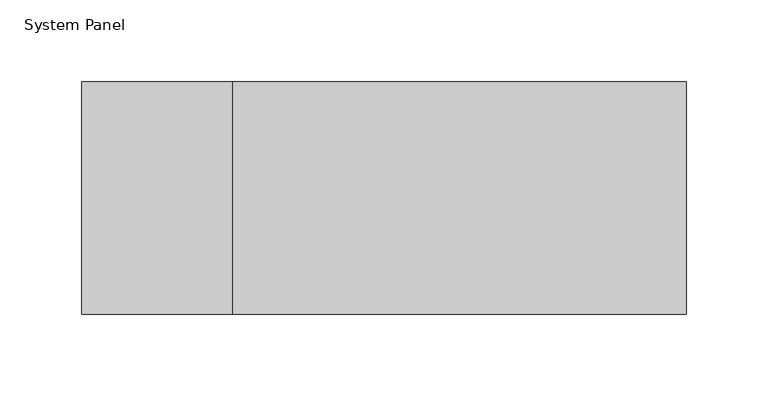
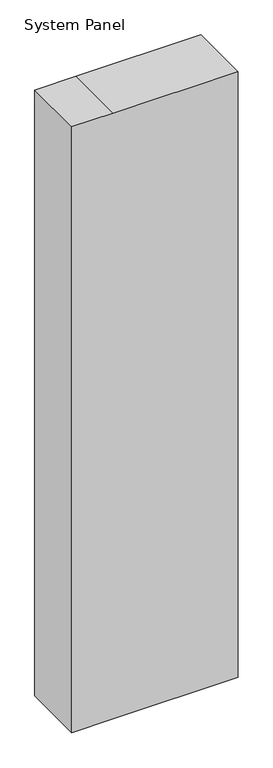
"""IFC4 building model written with IfcOpenShell, lengths in millimetres: plate geometry, System Panel : NLRS_21_CWP_hsb-vulling minerale wol 142 _gen_rsf."""

from ifc_helpers import new_model, si_unit, frame, origin, place, context, project, spatial, polyline, outline, extrude, source, transform, mapped, element, save


def system_panel_113e5983(model_context):
    return source(origin(), model_context, "Body", "SweptSolid", [
        extrude(outline(polyline([(0.0, -184.5), (0.0, -92.5), (0.0, 184.5), (1421.0, 184.5), (1421.0, -92.5), (1421.0, -184.5), (0.0, -184.5)])), frame((0.0, -71.0, 0.0), z_axis=(0.0, 1.0, 0.0), x_axis=(0.0, 0.0, 1.0)), (0.0, 0.0, 1.0), 142.0),
    ])


if __name__ == "__main__":
    model = new_model("IFC4")
    model_context = context("Model", 3, world=origin())
    ifc_project = project(units=[si_unit("LENGTHUNIT", "METRE", prefix="MILLI")], contexts=[model_context])
    site = spatial("IfcSite", under=ifc_project)
    building = spatial("IfcBuilding", under=site)
    placement = place(None, origin())
    system_panel_shape = system_panel_113e5983(model_context)
    element("IfcPlate", 1, ObjectType="System Panel : NLRS_21_CWP_hsb-vulling minerale wol 142 _gen_rsf", at=placement, inside=building, context=model_context, shape_type="MappedRepresentation", body=[
        mapped(system_panel_shape, transform((0.0, 0.0, 0.0), x_axis=(1.0, 0.0, 0.0), y_axis=(0.0, 1.0, 0.0), z_axis=(0.0, 0.0, 1.0))),
    ])
    save(model, "model.ifc")

# Revit data of these elements
# Type "System Panel : NLRS_21_CWP_hsb-vulling minerale wol 142 _gen_rsf"
#   Export Type to IFC As = "IfcWall"
#   Type IfcGUID = "07M7mRoiH1CR8m_RSKIwpC"
#   Assembly Code = "21.23"
# Element 1 (IfcPlate, "System Panel : NLRS_21_CWP_hsb-vulling minerale wol 142 _gen_rsf")
#   Materials on its faces: "NLRS_m1_isolatie minerale wol_gen_rsf"
# Materials
#   "NLRS_m1_isolatie minerale wol_gen_rsf": class "M - Anorganische materialen", colour RGB 200 200 140, transparency 0, Keynote = "m1", Manufacturer = "Revit Standards Foundation", URL = "www.revitstandards.org", Description = "isolatie minerale wol", Cost = 0
